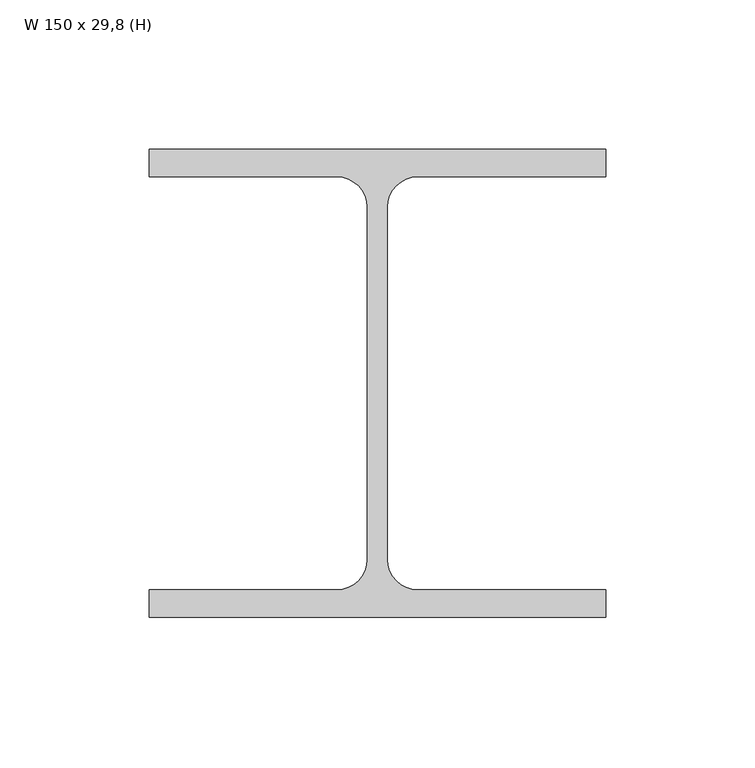
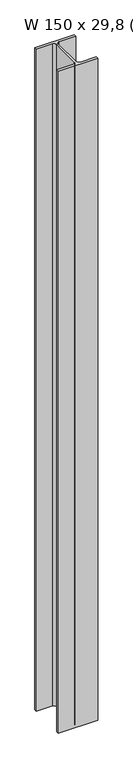
"""IFC4 building model written with IfcOpenShell, lengths in millimetres: column geometry, Pilar de Aço - H : W 150 x 29,8 (H)."""

from ifc_helpers import new_model, si_unit, point, frame_2d, origin, origin_with_axes, place, context, project, spatial, polyline, circle_curve, trimmed, segment, composite_curve, outline, extrude, source, transform, mapped, element, save


def w_150_x_29_8_h_a0631c91(model_context):
    return source(origin(), model_context, "Body", "SweptSolid", [
        extrude(outline(composite_curve([segment(polyline([(76.5, 78.5), (76.5, 69.2), (13.5, 69.2)]), True, "CONTINUOUS"), segment(trimmed(circle_curve(frame_2d((13.5, 59.0)), 10.2), [point((13.5, 69.2))], [point((3.3, 59.0))], True, "CARTESIAN"), True, "CONTINUOUS"), segment(polyline([(3.3, 59.0), (3.3, -59.0)]), True, "CONTINUOUS"), segment(trimmed(circle_curve(frame_2d((13.5, -59.0)), 10.2), [point((3.3, -59.0))], [point((13.5, -69.2))], True, "CARTESIAN"), True, "CONTINUOUS"), segment(polyline([(13.5, -69.2), (76.5, -69.2), (76.5, -78.5), (-76.5, -78.5), (-76.5, -69.2), (-13.5, -69.2)]), True, "CONTINUOUS"), segment(trimmed(circle_curve(frame_2d((-13.5, -59.0)), 10.2), [point((-13.5, -69.2))], [point((-3.3, -59.0))], True, "CARTESIAN"), True, "CONTINUOUS"), segment(polyline([(-3.3, -59.0), (-3.3, 59.0)]), True, "CONTINUOUS"), segment(trimmed(circle_curve(frame_2d((-13.5, 59.0)), 10.2), [point((-3.3, 59.0))], [point((-13.5, 69.2))], True, "CARTESIAN"), True, "CONTINUOUS"), segment(polyline([(-13.5, 69.2), (-76.5, 69.2), (-76.5, 78.5), (76.5, 78.5)]), True, "CONTINUOUS")], self_intersect=False)), origin_with_axes(), (0.0, 0.0, 1.0), 2720.0),
    ])


if __name__ == "__main__":
    model = new_model("IFC4")
    model_context = context("Model", 3, world=origin())
    ifc_project = project(units=[si_unit("LENGTHUNIT", "METRE", prefix="MILLI")], contexts=[model_context])
    site = spatial("IfcSite", under=ifc_project)
    building = spatial("IfcBuilding", under=site)
    placement = place(None, origin())
    w_150_x_29_8_h_shape = w_150_x_29_8_h_a0631c91(model_context)
    element("IfcColumn", 1, ObjectType="Pilar de Aço - H : W 150 x 29,8 (H)", at=placement, inside=building, context=model_context, shape_type="MappedRepresentation", body=[
        mapped(w_150_x_29_8_h_shape, transform((0.0, 0.0, 0.0), x_axis=(1.0, 0.0, 0.0), y_axis=(0.0, 1.0, 0.0), z_axis=(0.0, 0.0, 1.0))),
    ])
    save(model, "model.ifc")

# Revit data of these elements
# Type "Pilar de Aço - H : W 150 x 29,8 (H)"
#   SINAPI = ""
#   Área da seção = 38.5 m²
#   tw = 0.66 cm
#   tf = 0.93 cm
#   h = 13.84 cm
#   d' = 11.80 cm
#   d = 15.70 cm
#   bf = 15.30 cm
#   R = 1.02 cm
#   Massa Linear kg/m = 29.8
#   Aço = Metal - Aço 345MPa
#   Assembly Code = ""
# Materials
#   "Metal - Aço 345MPa": class "Metal", colour RGB 189 187 185, transparency 0, Cost = 0
